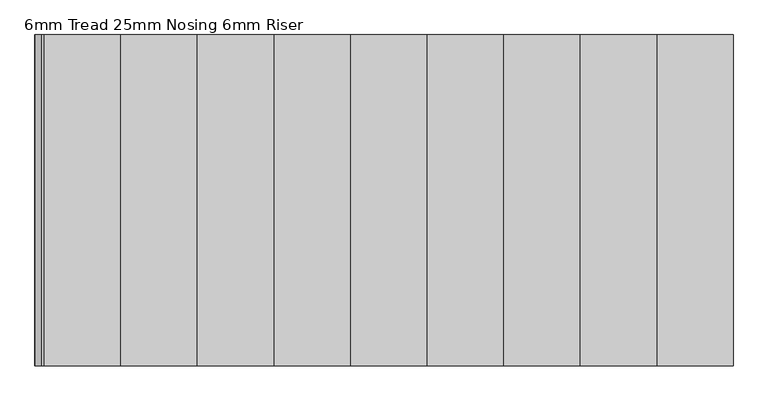
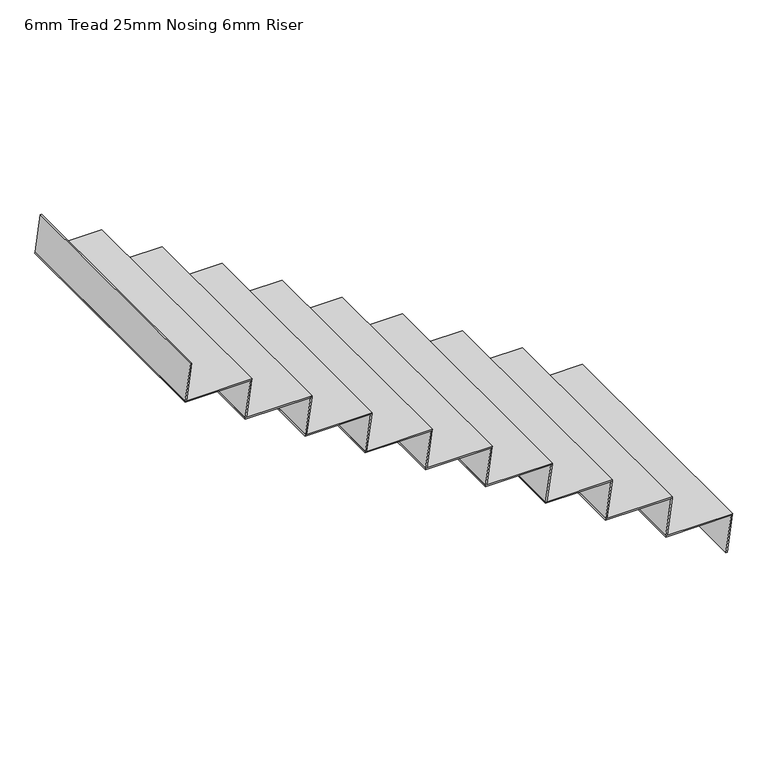
"""IFC4 building model written with IfcOpenShell, lengths in millimetres: stair flight geometry, 6mm Tread 25mm Nosing 6mm Riser."""

from ifc_helpers import new_model, si_unit, frame, origin, place, context, project, spatial, polyline, outline, extrude, source, transform, mapped, element, save


def stair_flight_6mm_tread_25mm_nosing_6mm_riser_1821247c(model_context):
    return source(origin(), model_context, "Body", "SweptSolid", [
        extrude(outline(polyline([(6400.0, 16350.0), (6400.0, 16043.9409643), (6394.0, 16043.0972143), (6394.0, 16349.15625), (6400.0, 16350.0)])), frame((0.0, 12030.4345331, 0.0), z_axis=(0.0, 1.0, 0.0), x_axis=(0.0, 0.0, 1.0)), (0.0, 0.0, 1.0), 1190.0),
        extrude(outline(polyline([(6394.0, 16349.15625), (6394.0, 16343.0972143), (6222.2222222, 16318.9409643), (6222.2222222, 16325.0), (6394.0, 16349.15625)])), frame((0.0, 12030.4345331, 0.0), z_axis=(0.0, 1.0, 0.0), x_axis=(0.0, 0.0, 1.0)), (0.0, 0.0, 1.0), 1190.0),
        extrude(outline(polyline([(6571.7777778, 16074.15625), (6571.7777778, 16068.0972143), (6400.0, 16043.9409643), (6400.0, 16050.0), (6571.7777778, 16074.15625)])), frame((0.0, 12030.4345331, 0.0), z_axis=(0.0, 1.0, 0.0), x_axis=(0.0, 0.0, 1.0)), (0.0, 0.0, 1.0), 1190.0),
        extrude(outline(polyline([(6577.7777778, 16075.0), (6577.7777778, 15768.9409643), (6571.7777778, 15768.0972143), (6571.7777778, 16074.15625), (6577.7777778, 16075.0)])), frame((0.0, 12030.4345331, 0.0), z_axis=(0.0, 1.0, 0.0), x_axis=(0.0, 0.0, 1.0)), (0.0, 0.0, 1.0), 1190.0),
        extrude(outline(polyline([(6749.5555556, 15799.15625), (6749.5555556, 15793.0972143), (6577.7777778, 15768.9409643), (6577.7777778, 15775.0), (6749.5555556, 15799.15625)])), frame((0.0, 12030.4345331, 0.0), z_axis=(0.0, 1.0, 0.0), x_axis=(0.0, 0.0, 1.0)), (0.0, 0.0, 1.0), 1190.0),
        extrude(outline(polyline([(6755.5555556, 15800.0), (6755.5555556, 15493.9409643), (6749.5555556, 15493.0972143), (6749.5555556, 15799.15625), (6755.5555556, 15800.0)])), frame((0.0, 12030.4345331, 0.0), z_axis=(0.0, 1.0, 0.0), x_axis=(0.0, 0.0, 1.0)), (0.0, 0.0, 1.0), 1190.0),
        extrude(outline(polyline([(6927.3333333, 15524.15625), (6927.3333333, 15518.0972143), (6755.5555556, 15493.9409643), (6755.5555556, 15500.0), (6927.3333333, 15524.15625)])), frame((0.0, 12030.4345331, 0.0), z_axis=(0.0, 1.0, 0.0), x_axis=(0.0, 0.0, 1.0)), (0.0, 0.0, 1.0), 1190.0),
        extrude(outline(polyline([(6933.3333333, 15525.0), (6933.3333333, 15218.9409643), (6927.3333333, 15218.0972143), (6927.3333333, 15524.15625), (6933.3333333, 15525.0)])), frame((0.0, 12030.4345331, 0.0), z_axis=(0.0, 1.0, 0.0), x_axis=(0.0, 0.0, 1.0)), (0.0, 0.0, 1.0), 1190.0),
        extrude(outline(polyline([(7105.1111111, 15249.15625), (7105.1111111, 15243.0972143), (6933.3333333, 15218.9409643), (6933.3333333, 15225.0), (7105.1111111, 15249.15625)])), frame((0.0, 12030.4345331, 0.0), z_axis=(0.0, 1.0, 0.0), x_axis=(0.0, 0.0, 1.0)), (0.0, 0.0, 1.0), 1190.0),
        extrude(outline(polyline([(7111.1111111, 15250.0), (7111.1111111, 14943.9409643), (7105.1111111, 14943.0972143), (7105.1111111, 15249.15625), (7111.1111111, 15250.0)])), frame((0.0, 12030.4345331, 0.0), z_axis=(0.0, 1.0, 0.0), x_axis=(0.0, 0.0, 1.0)), (0.0, 0.0, 1.0), 1190.0),
        extrude(outline(polyline([(7282.8888889, 14974.15625), (7282.8888889, 14968.0972143), (7111.1111111, 14943.9409643), (7111.1111111, 14950.0), (7282.8888889, 14974.15625)])), frame((0.0, 12030.4345331, 0.0), z_axis=(0.0, 1.0, 0.0), x_axis=(0.0, 0.0, 1.0)), (0.0, 0.0, 1.0), 1190.0),
        extrude(outline(polyline([(7288.8888889, 14975.0), (7288.8888889, 14668.9409643), (7282.8888889, 14668.0972143), (7282.8888889, 14974.15625), (7288.8888889, 14975.0)])), frame((0.0, 12030.4345331, 0.0), z_axis=(0.0, 1.0, 0.0), x_axis=(0.0, 0.0, 1.0)), (0.0, 0.0, 1.0), 1190.0),
        extrude(outline(polyline([(7460.6666667, 14699.15625), (7460.6666667, 14693.0972143), (7288.8888889, 14668.9409643), (7288.8888889, 14675.0), (7460.6666667, 14699.15625)])), frame((0.0, 12030.4345331, 0.0), z_axis=(0.0, 1.0, 0.0), x_axis=(0.0, 0.0, 1.0)), (0.0, 0.0, 1.0), 1190.0),
        extrude(outline(polyline([(7466.6666667, 14700.0), (7466.6666667, 14393.9409643), (7460.6666667, 14393.0972143), (7460.6666667, 14699.15625), (7466.6666667, 14700.0)])), frame((0.0, 12030.4345331, 0.0), z_axis=(0.0, 1.0, 0.0), x_axis=(0.0, 0.0, 1.0)), (0.0, 0.0, 1.0), 1190.0),
        extrude(outline(polyline([(7638.4444444, 14424.15625), (7638.4444444, 14418.0972143), (7466.6666667, 14393.9409643), (7466.6666667, 14400.0), (7638.4444444, 14424.15625)])), frame((0.0, 12030.4345331, 0.0), z_axis=(0.0, 1.0, 0.0), x_axis=(0.0, 0.0, 1.0)), (0.0, 0.0, 1.0), 1190.0),
        extrude(outline(polyline([(7644.4444444, 14425.0), (7644.4444444, 14118.9409643), (7638.4444444, 14118.0972143), (7638.4444444, 14424.15625), (7644.4444444, 14425.0)])), frame((0.0, 12030.4345331, 0.0), z_axis=(0.0, 1.0, 0.0), x_axis=(0.0, 0.0, 1.0)), (0.0, 0.0, 1.0), 1190.0),
        extrude(outline(polyline([(7816.2222222, 14149.15625), (7816.2222222, 14143.0972143), (7644.4444444, 14118.9409643), (7644.4444444, 14125.0), (7816.2222222, 14149.15625)])), frame((0.0, 12030.4345331, 0.0), z_axis=(0.0, 1.0, 0.0), x_axis=(0.0, 0.0, 1.0)), (0.0, 0.0, 1.0), 1190.0),
        extrude(outline(polyline([(7994.0, 13874.15625), (7994.0, 13868.0972143), (7822.2222222, 13843.9409643), (7822.2222222, 13850.0), (7994.0, 13874.15625)])), frame((0.0, 12030.4345331, 0.0), z_axis=(0.0, 1.0, 0.0), x_axis=(0.0, 0.0, 1.0)), (0.0, 0.0, 1.0), 1190.0),
        extrude(outline(polyline([(7822.2222222, 14150.0), (7822.2222222, 13843.9409643), (7816.2222222, 13843.0972143), (7816.2222222, 14149.15625), (7822.2222222, 14150.0)])), frame((0.0, 12030.4345331, 0.0), z_axis=(0.0, 1.0, 0.0), x_axis=(0.0, 0.0, 1.0)), (0.0, 0.0, 1.0), 1190.0),
    ])


if __name__ == "__main__":
    model = new_model("IFC4")
    model_context = context("Model", 3, world=origin())
    ifc_project = project(units=[si_unit("LENGTHUNIT", "METRE", prefix="MILLI")], contexts=[model_context])
    site = spatial("IfcSite", under=ifc_project)
    building = spatial("IfcBuilding", under=site)
    placement = place(None, origin())
    stair_flight_6mm_tread_25mm_nosing_6mm_riser_shape = stair_flight_6mm_tread_25mm_nosing_6mm_riser_1821247c(model_context)
    element("IfcStairFlight", 1, ObjectType="6mm Tread 25mm Nosing 6mm Riser", at=placement, inside=building, context=model_context, shape_type="MappedRepresentation", body=[
        mapped(stair_flight_6mm_tread_25mm_nosing_6mm_riser_shape, transform((0.0, 0.0, 0.0), x_axis=(1.0, 0.0, 0.0), y_axis=(0.0, 1.0, 0.0), z_axis=(0.0, 0.0, 1.0))),
    ])
    save(model, "model.ifc")

# Revit data of these elements
# Element 1 (IfcStairFlight, "6mm Tread 25mm Nosing 6mm Riser")
#   Materials on its faces: "Steel, Paint Finish, Dark Gray"
# Materials
#   "Steel, Paint Finish, Dark Gray": class "Metal", colour RGB 89 89 89, transparency 0, Description = "Steel, paint finish, dark gray, glossy", Cost = 0
